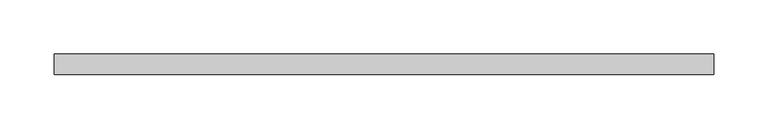
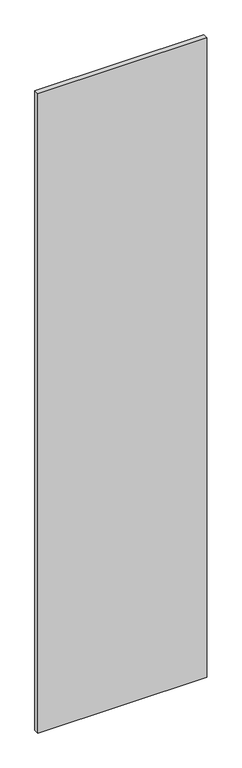
"""IFC4 building model written with IfcOpenShell, lengths in millimetres: proxy geometry, Vertical furring:Vertical furring:300288:Vertical furring:300288 : Vertical furring:Vertical furring:300288:300029:Vertical furring:300288:Vertical furring:300288 : Vertical furring:Vertical furring:300288:300029 : Vertical furring:Vertical furring:300288:Vertical furring:300288 : Vertical furring:Vertical furring:300288:300029:5 : Vertical furring:Vertical furring:300288:Vertical furring:300288 : Vertical furring:Vertical furring:300288:300029:Vertical furring:300288:Vertical furring:300288 : Vertical furring:Vertical furring:300288:300029 : Vertical furring:Vertical furring:300288:Vertical furring:300288 : Vertical furring:Vertical furring:300288:300029:300008."""

from ifc_helpers import new_model, si_unit, origin, origin_with_axes, place, context, project, spatial, polyline, outline, extrude, source, transform, mapped, element, save


def generic_models_25a56952(model_context):
    return source(origin(), model_context, "Body", "SweptSolid", [
        extrude(outline(polyline([(570452.6367239, -579070.5413841), (571062.2367239, -579070.5413841), (571062.2367239, -579089.5913841), (570452.6367239, -579089.5913841), (570452.6367239, -579070.5413841)])), origin_with_axes(), (0.0, 0.0, 1.0), 2438.4),
    ])


if __name__ == "__main__":
    model = new_model("IFC4")
    model_context = context("Model", 3, world=origin())
    ifc_project = project(units=[si_unit("LENGTHUNIT", "METRE", prefix="MILLI")], contexts=[model_context])
    site = spatial("IfcSite", under=ifc_project)
    building = spatial("IfcBuilding", under=site)
    placement = place(None, origin())
    generic_models_shape = generic_models_25a56952(model_context)
    element("IfcBuildingElementProxy", 1, Name="Vertical furring:Vertical furring:300288:Vertical furring:300288 : Vertical furring:Vertical furring:300288:300029:Vertical furring:300288:Vertical furring:300288 : Vertical furring:Vertical furring:300288:300029 : Vertical furring:Vertical furring:300288:Vertical furring:300288 : Vertical furring:Vertical furring:300288:300029:5 : Vertical furring:Vertical furring:300288:Vertical furring:300288 : Vertical furring:Vertical furring:300288:300029:Vertical furring:300288:Vertical furring:300288 : Vertical furring:Vertical furring:300288:300029 : Vertical furring:Vertical furring:300288:Vertical furring:300288 : Vertical furring:Vertical furring:300288:300029:300008", ObjectType="Vertical furring:Vertical furring:300288:Vertical furring:300288 : Vertical furring:Vertical furring:300288:300029:Vertical furring:300288:Vertical furring:300288 : Vertical furring:Vertical furring:300288:300029 : Vertical furring:Vertical furring:300288:Vertical furring:300288 : Vertical furring:Vertical furring:300288:300029:5 : Vertical furring:Vertical furring:300288:Vertical furring:300288 : Vertical furring:Vertical furring:300288:300029:Vertical furring:300288:Vertical furring:300288 : Vertical furring:Vertical furring:300288:300029 : Vertical furring:Vertical furring:300288:Vertical furring:300288 : Vertical furring:Vertical furring:300288:300029:300008", at=placement, inside=building, context=model_context, shape_type="MappedRepresentation", body=[
        mapped(generic_models_shape, transform((0.0, 0.0, 0.0), x_axis=(1.0, 0.0, 0.0), y_axis=(0.0, 1.0, 0.0), z_axis=(0.0, 0.0, 1.0))),
    ])
    save(model, "model.ifc")

# Revit data of these elements
# Type "Vertical furring:Vertical furring:300288:Vertical furring:300288 : Vertical furring:Vertical furring:300288:300029:Vertical furring:300288:Vertical furring:300288 : Vertical furring:Vertical furring:300288:300029 : Vertical furring:Vertical furring:300288:Vertical furring:300288 : Vertical furring:Vertical furring:300288:300029:5 : Vertical furring:Vertical furring:300288:Vertical furring:300288 : Vertical furring:Vertical furring:300288:300029:Vertical furring:300288:Vertical furring:300288 : Vertical furring:Vertical furring:300288:300029 : Vertical furring:Vertical furring:300288:Vertical furring:300288 : Vertical furring:Vertical furring:300288:300029:300008"
#   NameOverride = "Vertical furring:Vertical furring:300288:Vertical furring:300288 : Vertical furring:Vertical furring:300288:300029:Vertical furring:300288:Vertical furring:300288 : Vertical furring:Vertical furring:300288:300029 : Vertical furring:Vertical furring:300288:Vertical furring:300288 : Vertical furring:Vertical furring:300288:300029:300008"
#   ObjectTypeOverride = "Vertical furring:300288:Vertical furring:300288 : Vertical furring:Vertical furring:300288:300029 : Vertical furring:Vertical furring:300288:Vertical furring:300288 : Vertical furring:Vertical furring:300288:300029"
#   Reference = "Vertical furring"
#   Tag = "300008"
# Element 1 (IfcBuildingElementProxy, "Vertical furring:Vertical furring:300288:Vertical furring:300288 : Vertical furring:Vertical furring:300288:300029:Vertical furring:300288:Vertical furring:300288 : Vertical furring:Vertical furring:300288:300029 : Vertical furring:Vertical furring:300288:Vertical furring:300288 : Vertical furring:Vertical furring:300288:300029:5 : Vertical furring:Vertical furring:300288:Vertical furring:300288 : Vertical furring:Vertical furring:300288:300029:Vertical furring:300288:Vertical furring:300288 : Vertical furring:Vertical furring:300288:300029 : Vertical furring:Vertical furring:300288:Vertical furring:300288 : Vertical furring:Vertical furring:300288:300029:300008")
#   Materials on its faces: "1\" MINERAL WOOL BOARD INSULATION"
# Materials
#   "1\" MINERAL WOOL BOARD INSULATION": class "Unassigned", colour RGB 205 188 106, transparency 0, Cost = 0
